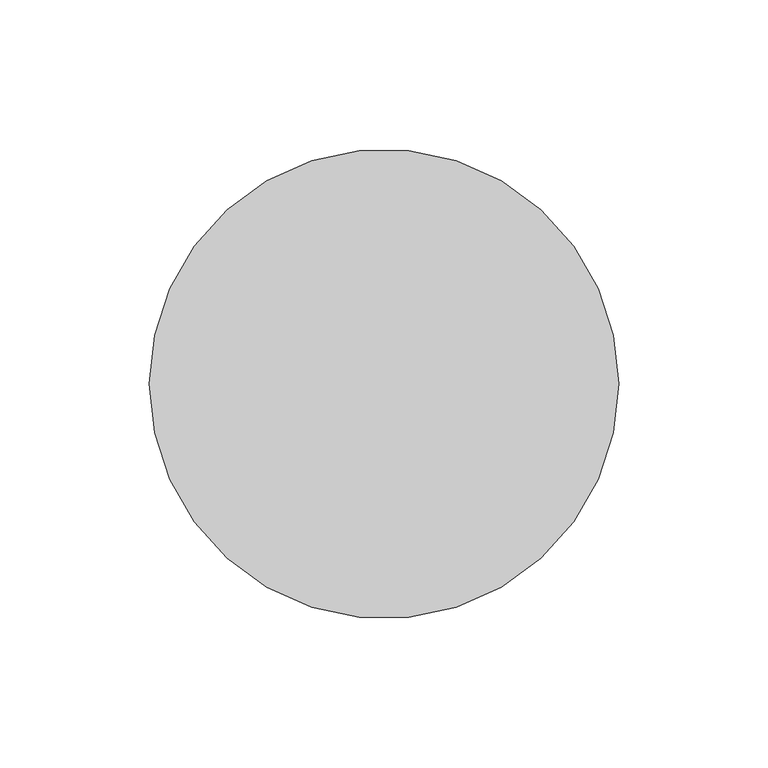
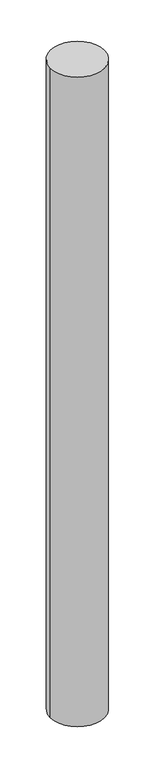
"""IFC4 building model written with IfcOpenShell, lengths in millimetres: proxy geometry, NLRS_71_GM_WPB_afschermpaal aardebaan_gen_rsf : afschermpaal aardebaan dxl 159x2000mm."""

from ifc_helpers import new_model, si_unit, point, frame, frame_2d, origin, place, context, project, spatial, circle_curve, trimmed, segment, composite_curve, outline, extrude, source, transform, mapped, element, save


def generic_models_0e34d4cd(model_context):
    return source(origin(), model_context, "Body", "SweptSolid", [
        extrude(outline(composite_curve([segment(trimmed(circle_curve(frame_2d((1.2, 75.0)), 78.5), [point((-77.3, 75.0))], [point((79.7, 75.0))], False, "CARTESIAN"), True, "CONTINUOUS"), segment(trimmed(circle_curve(frame_2d((1.2, 75.0)), 78.5), [point((79.7, 75.0))], [point((-77.3, 75.0))], False, "CARTESIAN"), True, "CONTINUOUS")], self_intersect=False)), frame((0.0, 0.0, -1000.0), z_axis=(0.0, 0.0, 1.0), x_axis=(1.0, 0.0, 0.0)), (0.0, 0.0, 1.0), 2000.0),
    ])


if __name__ == "__main__":
    model = new_model("IFC4")
    model_context = context("Model", 3, world=origin())
    ifc_project = project(units=[si_unit("LENGTHUNIT", "METRE", prefix="MILLI")], contexts=[model_context])
    site = spatial("IfcSite", under=ifc_project)
    building = spatial("IfcBuilding", under=site)
    placement = place(None, origin())
    generic_models_shape = generic_models_0e34d4cd(model_context)
    element("IfcBuildingElementProxy", 1, Name="NLRS_71_GM_WPB_afschermpaal aardebaan_gen_rsf : afschermpaal aardebaan dxl 159x2000mm", ObjectType="NLRS_71_GM_WPB_afschermpaal aardebaan_gen_rsf : afschermpaal aardebaan dxl 159x2000mm", at=placement, inside=building, context=model_context, shape_type="MappedRepresentation", body=[
        mapped(generic_models_shape, transform((0.0, 0.0, 0.0), x_axis=(1.0, 0.0, 0.0), y_axis=(0.0, 1.0, 0.0), z_axis=(0.0, 0.0, 1.0))),
    ])
    save(model, "model.ifc")

# Revit data of these elements
# Type "NLRS_71_GM_WPB_afschermpaal aardebaan_gen_rsf : afschermpaal aardebaan dxl 159x2000mm"
#   Type IFC Predefined Type = "USERDEFINED"
#   Export Type to IFC As = "IfcGeographicElementType"
#   Type IfcGUID = "05J6pyYiTDtR2exmlhyPlb"
#   IfcName[Type] = "afschermpaal aardebaan dxl 159x2000mm"
#   IfcDescription[Type] = "verkeerspaal dxl 159x2000mm"
#   IfcObjectType[Type] = "BOLLARD"
#   IfcExportAs[Type] = "IfcGeographicElementType"
#   IfcExportType[Type] = "USERDEFINED"
#   NLRS_C_revit_versie = "2021"
#   NLRS_C_materiaal_afwerking [instance default] = ""
#   NLRS_C_content_versie = ""
#   NLRS_C_content_provider = ""
#   NLRS_C_content_handleiding = ""
#   NLRS_C_content_datum_uitgifte = ""
#   NLRS_C_content_datum_gewijzigd = ""
#   NLRS_C_content_creator = ""
#   NLRS_C_brandwerendheid_text [instance default] = ""
#   NLRS_C_brandwerendheid_EI_text [instance default] = ""
#   Model = "generiek"
#   Manufacturer = "generiek"
#   Description = "verkeerspaal dxl 159x2000mm"
#   Assembly Code = "71.10"
#   NLRS_S_gewicht [instance default] = 0.00 kg
#   NLRS_C_radius = 78.50 mm
#   NLRS_C_offset [instance default] = 0.00 mm
#   NLRS_C_hoogte = 2000.00 mm
#   NLRS_C_diepte = 1000.00 mm
#   NLRS_C_buiten [instance default] = yes
#   NLRS_C_brandwerend [instance default] = yes
#   NLRS_C_brandbaar [instance default] = yes
#   NLRS_C_materiaal = none
#   URL = ""
#   Default Elevation = 0
# Element 1 (IfcBuildingElementProxy, "NLRS_71_GM_WPB_afschermpaal aardebaan_gen_rsf : afschermpaal aardebaan dxl 159x2000mm")
#   NLRS_C_offset = 344.718 mm
